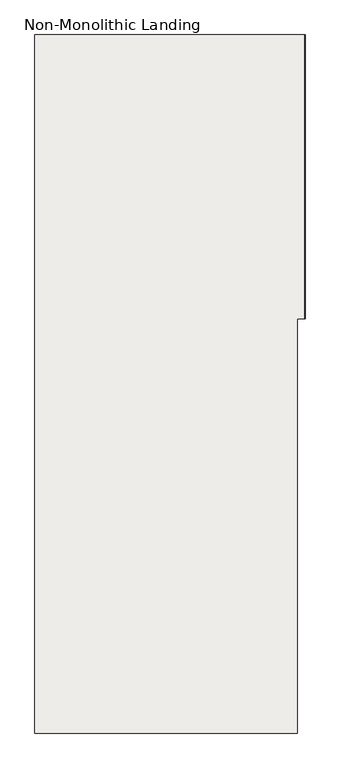
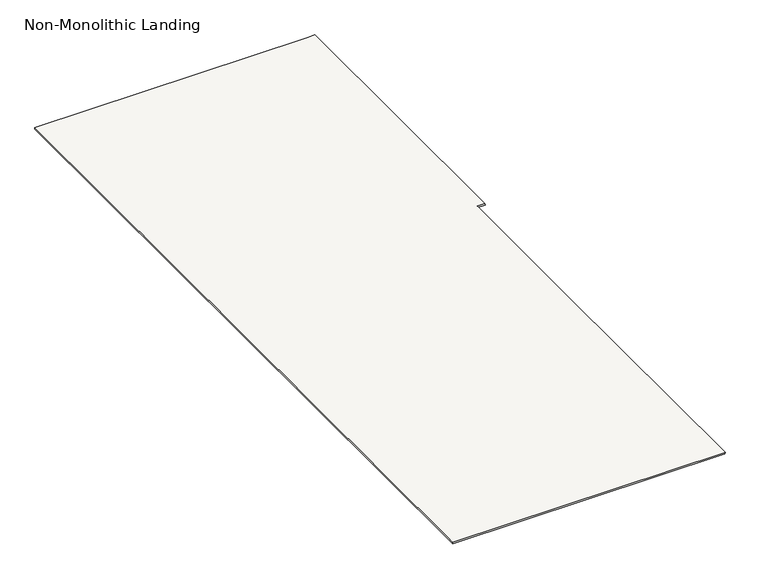
"""IFC4 building model written with IfcOpenShell, lengths in millimetres: slab geometry, Non-Monolithic Landing."""

from ifc_helpers import new_model, si_unit, origin, place, context, project, spatial, faceted_brep, source, transform, mapped, element, save


def non_monolithic_landing_a73df6c7(model_context):
    return source(origin(), model_context, "Body", "Brep", [
        faceted_brep([(-16318.9400908, 12030.4345331, 26352.9411765), (-16318.0900908, 12030.4345331, 26346.9411765), (-16318.0900908, 13220.4345331, 26346.9411765), (-16318.9400908, 13220.4345331, 26352.9411765), (-16350.0, 11395.4345331, 26352.9411765), (-16350.0, 12030.4345331, 26352.9411765), (-16350.0, 13220.4345331, 26352.9411765), (-17450.0, 13220.4345331, 26352.9411765), (-17450.0, 10295.4345331, 26352.9411765), (-16350.0, 10295.4345331, 26352.9411765), (-16350.0, 12030.4345331, 26346.9411765), (-16350.0, 11395.4345331, 26346.9411765), (-16350.85, 11395.4345331, 26346.9411765), (-16350.85, 10295.4345331, 26346.9411765), (-17450.0, 10295.4345331, 26346.9411765), (-17450.0, 13220.4345331, 26346.9411765), (-16350.0, 13220.4345331, 26346.9411765)], [[[0, 1, 2, 3]], [[4, 5, 0, 3, 6, 7, 8, 9]], [[10, 11, 12, 13, 14, 15, 16, 2, 1]], [[5, 4, 11, 10]], [[0, 5, 10, 1]], [[6, 3, 2, 16]], [[7, 6, 16, 15]], [[8, 7, 15, 14]], [[9, 8, 14, 13]], [[4, 12, 11]], [[12, 4, 9, 13]]]),
    ])


if __name__ == "__main__":
    model = new_model("IFC4")
    model_context = context("Model", 3, world=origin())
    ifc_project = project(units=[si_unit("LENGTHUNIT", "METRE", prefix="MILLI")], contexts=[model_context])
    site = spatial("IfcSite", under=ifc_project)
    building = spatial("IfcBuilding", under=site)
    placement = place(None, origin())
    non_monolithic_landing_shape = non_monolithic_landing_a73df6c7(model_context)
    element("IfcSlab", 1, ObjectType="Non-Monolithic Landing", at=placement, inside=building, context=model_context, shape_type="MappedRepresentation", body=[
        mapped(non_monolithic_landing_shape, transform((0.0, 0.0, 0.0), x_axis=(1.0, 0.0, 0.0), y_axis=(0.0, 1.0, 0.0), z_axis=(0.0, 0.0, 1.0))),
    ])
    save(model, "model.ifc")

# Revit data of these elements
# Element 1 (IfcSlab, "Non-Monolithic Landing")
#   Materials on its faces: "Steel, Paint Finish, Dark Gray"
# Materials
#   "Steel, Paint Finish, Dark Gray": class "Metal", colour RGB 89 89 89, transparency 0, Description = "Steel, paint finish, dark gray, glossy", Cost = 0
